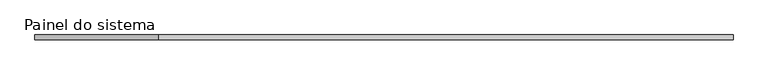
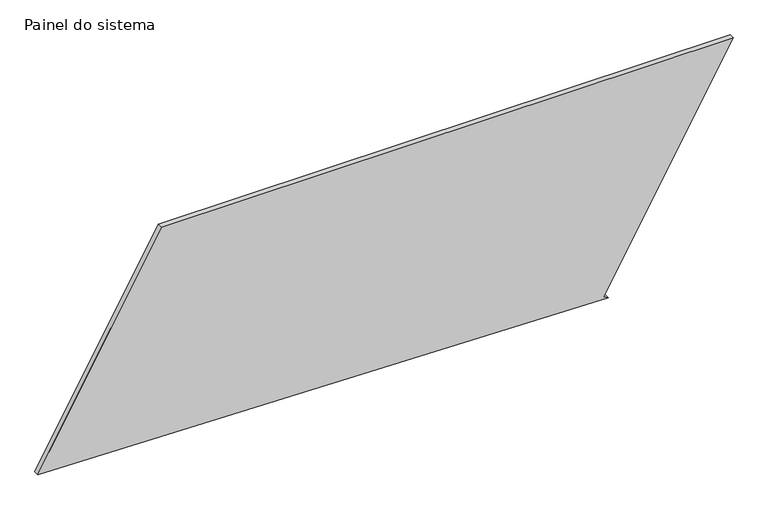
"""IFC4 building model written with IfcOpenShell, lengths in millimetres: plate geometry, Painel do sistema : Envidraçado."""

from ifc_helpers import new_model, si_unit, frame, origin, place, context, project, spatial, polyline, outline, extrude, source, transform, mapped, element, save


def painel_do_sistema_161353ff(model_context):
    return source(origin(), model_context, "Body", "SweptSolid", [
        extrude(outline(polyline([(0.0, 1139.4275543), (12.2820845, 1117.6525595), (1182.489881, 1777.7028244), (1182.489881, -1147.2450056), (64.7467421, -1777.7028244), (0.0, 1139.4275543)])), frame((0.0, 24.5, 0.0), z_axis=(0.0, 1.0, 0.0), x_axis=(0.0, 0.0, 1.0)), (0.0, 0.0, 1.0), 25.0),
    ])


if __name__ == "__main__":
    model = new_model("IFC4")
    model_context = context("Model", 3, world=origin())
    ifc_project = project(units=[si_unit("LENGTHUNIT", "METRE", prefix="MILLI")], contexts=[model_context])
    site = spatial("IfcSite", under=ifc_project)
    building = spatial("IfcBuilding", under=site)
    placement = place(None, origin())
    painel_do_sistema_shape = painel_do_sistema_161353ff(model_context)
    element("IfcPlate", 1, ObjectType="Painel do sistema : Envidraçado", at=placement, inside=building, context=model_context, shape_type="MappedRepresentation", body=[
        mapped(painel_do_sistema_shape, transform((0.0, 0.0, 0.0), x_axis=(1.0, 0.0, 0.0), y_axis=(0.0, 1.0, 0.0), z_axis=(0.0, 0.0, 1.0))),
    ])
    save(model, "model.ifc")

# Revit data of these elements
# Type "Painel do sistema : Envidraçado"
#   Construction Type Id = "GSP4R"
#   Analytic Construction = "Vidraça única Pilkington 1/8 pol"
#   Visual Light Transmittance = 0.9
#   Solar Heat Gain Coefficient = 0.86
#   Heat Transfer Coefficient (U) = 6.7069 W/(m²·K)
# Element 1 (IfcPlate, "Painel do sistema : Envidraçado")
#   Materials on its faces: "Vidro"
# Materials
#   "Vidro": class "Vidro", colour RGB 0 128 192, transparency 0.9, Description = "Vidro de sílica", Cost = 0
